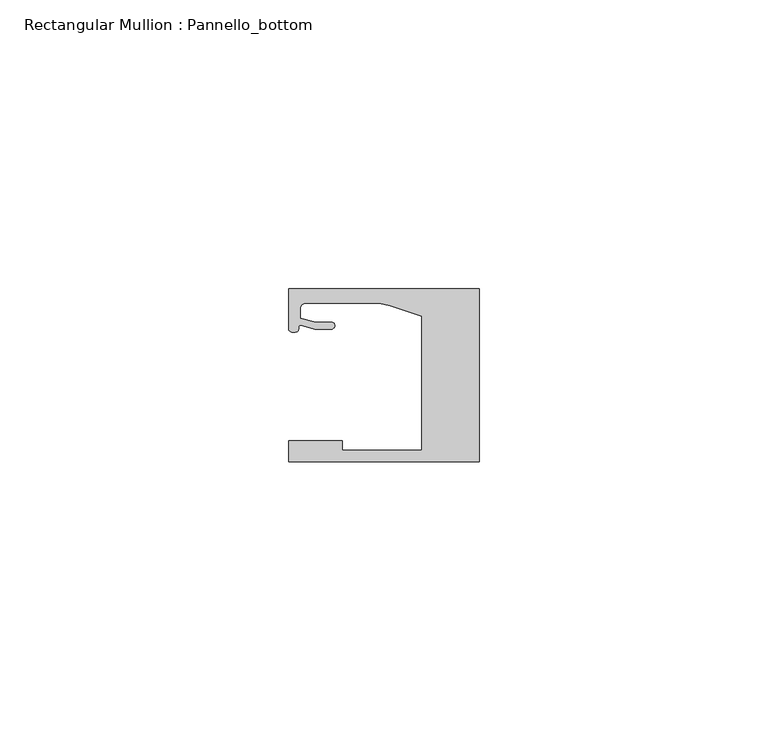
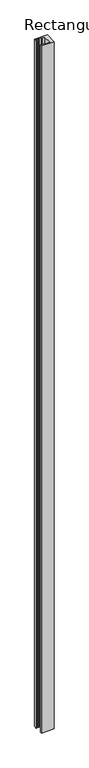
"""IFC4 building model written with IfcOpenShell, lengths in millimetres: member geometry, Rectangular Mullion : Pannello_bottom."""

from ifc_helpers import new_model, si_unit, frame, origin, place, context, project, spatial, polyline, circle_curve, source, transform, mapped, element, save
from ifc_brep_helpers import plane_surface, cylinder_surface, revolved_surface, extruded_surface, spline_curve, advanced_brep


def rectangular_mullion_pannello_bottom_55b4ac8b(model_context):
    return source(origin(), model_context, "Body", "AdvancedBrep", [
        advanced_brep(
        [(-33.0, -15.0, 0.0), (0.0, -15.0, 0.0), (0.0, 15.0, 0.0), (-33.0000135, 15.0, 0.0), (-33.0000135, 8.0000472, 0.0), (-30.9223017, 8.6490241, 0.0), (-28.4999305, 7.9999523, 0.0), (-25.59998, 7.9999523, 0.0), (-25.59998, 9.1999523, 0.0), (-28.3419477, 9.1999523, 0.0), (-31.0, 9.9121746, 0.0), (-31.0, 11.4999419, 0.0), (-30.0000002, 12.4999419, 0.0), (-18.5493024, 12.4999438, 0.0), (-15.4591336, 12.0105099, 0.0), (-9.9999723, 10.2367227, 0.0), (-9.9999723, -13.0000004, 0.0), (-23.700041, -13.0000004, 0.0), (-23.700041, -11.3000004, 0.0), (-33.0, -11.3000004, 0.0), (-33.0, -15.0, -1883.9999729), (-33.0, -11.3000004, -1883.9999729), (-23.700041, -11.3000004, -1883.9999729), (-23.700041, -13.0000004, -1883.9999729), (-9.9999723, -13.0000004, -1883.9999729), (-9.9999723, 10.2367227, -1883.9999729), (-15.4591336, 12.0105099, -1883.9999729), (-18.5493024, 12.4999438, -1883.9999729), (-30.0000002, 12.4999419, -1883.9999729), (-31.0, 11.4999419, -1883.9999729), (-31.0, 9.9121746, -1883.9999729), (-28.3419477, 9.1999523, -1883.9999729), (-25.59998, 9.1999523, -1883.9999729), (-25.59998, 7.9999523, -1883.9999729), (-28.4999305, 7.9999523, -1883.9999729), (-30.9223017, 8.6490241, -1883.9999729), (-33.0000135, 8.0000472, -1883.9999729), (-33.0000135, 15.0, -1883.9999729), (0.0, 15.0, -1883.9999729), (0.0, -15.0, -1883.9999729)],
        [
            (0, 1),
            (1, 2),
            (2, 3),
            (3, 4),
            (4, 5, spline_curve(3, [(-33.0000135, 8.0000472, 0.0), (-33.0000135, 7.457047519, 0.0), (-32.262327879, 7.456527435, 0.0), (-31.357433266, 7.563996614, 0.0), (-31.305645054, 7.690065204, 0.0), (-31.298563602, 8.366228555, 0.0), (-31.312054066, 8.717747958, 0.0), (-30.9223017, 8.6490241, 0.0)], [4, 2, 2, 4], [0.0, 0.0027053965905959043, 0.0058611956533709, 0.007702013405570312])),
            (5, 6),
            (6, 7),
            (7, 8, circle_curve(frame((-25.59998, 8.5999523, 0.0), z_axis=(0.0, 0.0, 1.0), x_axis=(0.0, 1.0, 0.0)), 0.6)),
            (8, 9),
            (9, 10),
            (10, 11),
            (11, 12, circle_curve(frame((-30.0, 11.4999419, 0.0), z_axis=(0.0, 0.0, -1.0), x_axis=(0.0, 1.0, 0.0)), 1.0)),
            (12, 13),
            (13, 14, circle_curve(frame((-18.5493007, 2.4999438, 0.0), z_axis=(0.0, 0.0, -1.0), x_axis=(0.0, 1.0, 0.0)), 10.0)),
            (14, 15),
            (15, 16),
            (16, 17),
            (17, 18),
            (18, 19),
            (19, 0),
            (20, 21),
            (21, 22),
            (22, 23),
            (23, 24),
            (24, 25),
            (25, 26),
            (26, 27, circle_curve(frame((-18.5493007, 2.4999438, -1883.9999729), z_axis=(0.0, 0.0, 1.0), x_axis=(0.0, 1.0, 0.0)), 10.0)),
            (27, 28),
            (28, 29, circle_curve(frame((-30.0, 11.4999419, -1883.9999729), z_axis=(0.0, 0.0, 1.0), x_axis=(0.0, 1.0, 0.0)), 1.0)),
            (29, 30),
            (30, 31),
            (31, 32),
            (32, 33, circle_curve(frame((-25.59998, 8.5999523, -1883.9999729), z_axis=(0.0, 0.0, -1.0), x_axis=(0.0, 1.0, 0.0)), 0.6)),
            (33, 34),
            (34, 35),
            (35, 36, spline_curve(3, [(-30.9223017, 8.6490241, -1883.9999729), (-31.312054066, 8.717747958, -1883.9999729), (-31.298563602, 8.366228555, -1883.9999729), (-31.305645054, 7.690065204, -1883.9999729), (-31.357433266, 7.563996614, -1883.9999729), (-32.262327879, 7.456527435, -1883.9999729), (-33.0000135, 7.457047519, -1883.9999729), (-33.0000135, 8.0000472, -1883.9999729)], [4, 2, 2, 4], [0.0, 0.001840817752199412, 0.004996616814974408, 0.007702013405570312])),
            (36, 37),
            (37, 38),
            (38, 39),
            (39, 20),
            (0, 20),
            (39, 1),
            (38, 2),
            (37, 3),
            (36, 4),
            (35, 5),
            (34, 6),
            (33, 7),
            (32, 8),
            (31, 9),
            (30, 10),
            (29, 11),
            (28, 12),
            (27, 13),
            (26, 14),
            (25, 15),
            (24, 16),
            (23, 17),
            (22, 18),
            (21, 19),
        ],
        [
            plane_surface(frame((0.0, -36.2491502, 0.0), z_axis=(0.0, 0.0, 1.0), x_axis=(-1.0, 0.0, 0.0))),
            plane_surface(frame((0.0, -36.2491502, -1883.9999729), z_axis=(0.0, 0.0, -1.0), x_axis=(-1.0, 0.0, 0.0))),
            plane_surface(frame((-33.0, -15.0, 0.0), z_axis=(0.0, -1.0, 0.0), x_axis=(0.0, 0.0, -1.0))),
            plane_surface(frame((0.0, -15.0, 0.0), z_axis=(1.0, 0.0, 0.0), x_axis=(0.0, 0.0, -1.0))),
            plane_surface(frame((0.0, 15.0, 0.0), z_axis=(0.0, 1.0, 0.0), x_axis=(0.0, 0.0, -1.0))),
            plane_surface(frame((-33.0000135, 15.0, 0.0), z_axis=(-1.0, 0.0, 0.0), x_axis=(0.0, 0.0, -1.0))),
            extruded_surface(spline_curve(3, [(-33.0000135, 8.0000472, -1883.9999729), (-33.0000135, 7.457047519, -1883.9999729), (-32.262327879, 7.456527435, -1883.9999729), (-31.357433266, 7.563996614, -1883.9999729), (-31.305645054, 7.690065204, -1883.9999729), (-31.298563602, 8.366228555, -1883.9999729), (-31.312054066, 8.717747958, -1883.9999729), (-30.9223017, 8.6490241, -1883.9999729)], [4, 2, 2, 4], [0.0, 0.0027053965905959043, 0.0058611956533709, 0.007702013405570312]), (0.0, 0.0, 1883.9999729), 1883.9999729),
            plane_surface(frame((-30.9223017, 8.6490241, 0.0), z_axis=(-0.25881883200192934, -0.9659258833891746, 0.0), x_axis=(0.0, 0.0, -1.0))),
            plane_surface(frame((-28.4999305, 7.9999523, 0.0), z_axis=(0.0, -1.0, 0.0), x_axis=(0.0, 0.0, -1.0))),
            cylinder_surface(frame((-25.59998, 8.5999523, 0.0), z_axis=(0.0, 0.0, 1.0), x_axis=(0.0, 1.0, 0.0)), 0.6),
            plane_surface(frame((-25.59998, 9.1999523, 0.0), z_axis=(0.0, 1.0, 0.0), x_axis=(0.0, 0.0, -1.0))),
            plane_surface(frame((-28.3419477, 9.1999523, 0.0), z_axis=(0.25881883204288636, 0.9659258833782002, 0.0), x_axis=(0.0, 0.0, -1.0))),
            plane_surface(frame((-31.0, 9.9121746, 0.0), z_axis=(1.0, 0.0, 0.0), x_axis=(0.0, 0.0, -1.0))),
            revolved_surface(polyline([(-30.0, 12.4999419, -1883.9999729), (-30.0, 12.4999419, 0.0)]), (-30.0, 11.4999419, 0.0), (0.0, 0.0, -1.0)),
            plane_surface(frame((-30.0000002, 12.4999419, 0.0), z_axis=(1.6923026533778639e-07, -0.9999999999999858, 0.0), x_axis=(0.0, 0.0, -1.0))),
            revolved_surface(polyline([(-18.5493007, 12.4999438, -1883.9999729), (-18.5493007, 12.4999438, 0.0)]), (-18.5493007, 2.4999438, 0.0), (0.0, 0.0, -1.0)),
            plane_surface(frame((-15.4591336, 12.0105099, 0.0), z_axis=(-0.30901670911956314, -0.9510566089801992, 0.0), x_axis=(0.0, 0.0, -1.0))),
            plane_surface(frame((-9.9999723, 10.2367227, 0.0), z_axis=(-1.0, 0.0, 0.0), x_axis=(0.0, 0.0, -1.0))),
            plane_surface(frame((-9.9999723, -13.0000004, 0.0), z_axis=(0.0, 1.0, 0.0), x_axis=(0.0, 0.0, -1.0))),
            plane_surface(frame((-23.700041, -13.0000004, 0.0), z_axis=(1.0, 0.0, 0.0), x_axis=(0.0, 0.0, -1.0))),
            plane_surface(frame((-23.700041, -11.3000004, 0.0), z_axis=(0.0, 1.0, 0.0), x_axis=(0.0, 0.0, -1.0))),
            plane_surface(frame((-33.0, -11.3000004, 0.0), z_axis=(-1.0, 0.0, 0.0), x_axis=(0.0, 0.0, -1.0))),
        ],
        [
            (0, [[1, 2, 3, 4, 5, 6, 7, 8, 9, 10, 11, 12, 13, 14, 15, 16, 17, 18, 19, 20]]),
            (1, [[21, 22, 23, 24, 25, 26, 27, 28, 29, 30, 31, 32, 33, 34, 35, 36, 37, 38, 39, 40]]),
            (2, [[-1, 41, -40, 42]]),
            (3, [[-2, -42, -39, 43]]),
            (4, [[-3, -43, -38, 44]]),
            (5, [[-4, -44, -37, 45]]),
            (6, [[-5, -45, -36, 46]]),
            (7, [[-6, -46, -35, 47]]),
            (8, [[-7, -47, -34, 48]]),
            (9, [[-8, -48, -33, 49]]),
            (10, [[-9, -49, -32, 50]]),
            (11, [[-10, -50, -31, 51]]),
            (12, [[-11, -51, -30, 52]]),
            (13, [[-12, -52, -29, 53]]),
            (14, [[-13, -53, -28, 54]]),
            (15, [[-14, -54, -27, 55]]),
            (16, [[-15, -55, -26, 56]]),
            (17, [[-16, -56, -25, 57]]),
            (18, [[-17, -57, -24, 58]]),
            (19, [[-18, -58, -23, 59]]),
            (20, [[-19, -59, -22, 60]]),
            (21, [[-20, -60, -21, -41]]),
        ],
    ),
    ])


if __name__ == "__main__":
    model = new_model("IFC4")
    model_context = context("Model", 3, world=origin())
    ifc_project = project(units=[si_unit("LENGTHUNIT", "METRE", prefix="MILLI")], contexts=[model_context])
    site = spatial("IfcSite", under=ifc_project)
    building = spatial("IfcBuilding", under=site)
    placement = place(None, origin())
    rectangular_mullion_pannello_bottom_shape = rectangular_mullion_pannello_bottom_55b4ac8b(model_context)
    element("IfcMember", 1, ObjectType="Rectangular Mullion : Pannello_bottom", at=placement, inside=building, context=model_context, shape_type="MappedRepresentation", body=[
        mapped(rectangular_mullion_pannello_bottom_shape, transform((0.0, 0.0, 0.0), x_axis=(1.0, 0.0, 0.0), y_axis=(0.0, 1.0, 0.0), z_axis=(0.0, 0.0, 1.0))),
    ])
    save(model, "model.ifc")

# Revit data of these elements
# Type "Rectangular Mullion : Pannello_bottom"
#   built-in parameter 1007322 = 0.0984252 (stored number, unit not read)
#   built-in parameter 1007321 = 0.0328083 (stored number, unit not read)
#   built-in parameter 1007320 = 0 (stored number, unit not read)
